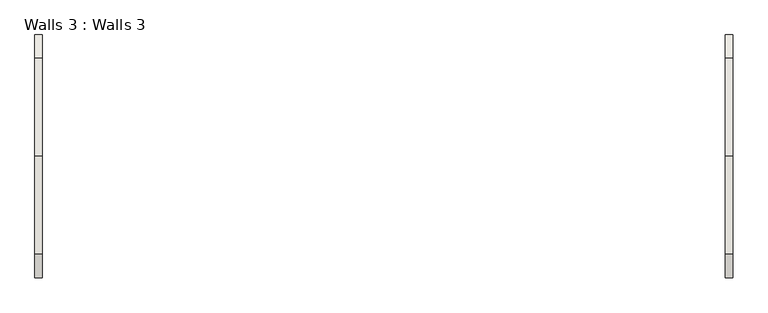
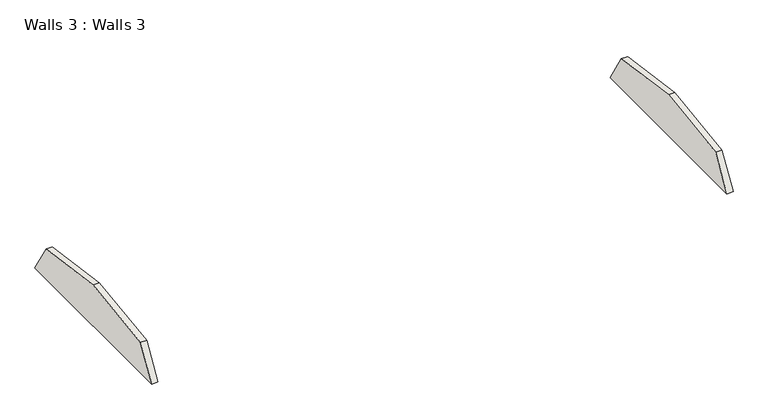
"""IFC4 building model written with IfcOpenShell, lengths in millimetres: wall geometry, Walls 3 : Walls 3."""

from ifc_helpers import new_model, si_unit, frame, origin, place, context, project, spatial, polyline, outline, extrude, source, transform, mapped, element, save


def walls_3_walls_3_da5502db(model_context):
    return source(origin(), model_context, "Body", "SweptSolid", [
        extrude(outline(polyline([(7113.2615366, 4718.0467955), (10133.2027784, 4305.4367595), (10859.8068451, 3111.5), (3366.7162281, 3111.5), (4093.3202949, 4305.4367595), (7113.2615366, 4718.0467955)])), frame((28804.3870052, 0.0, 0.0), z_axis=(1.0, 0.0, 0.0), x_axis=(0.0, 1.0, 0.0)), (0.0, 0.0, 1.0), 228.6),
        extrude(outline(polyline([(7113.2615366, 4718.0467955), (10133.2027784, 4305.4367595), (10859.8068451, 3111.5), (3366.7162281, 3111.5), (4093.3202949, 4305.4367595), (7113.2615366, 4718.0467955)])), frame((7500.1370052, 0.0, 0.0), z_axis=(1.0, 0.0, 0.0), x_axis=(0.0, 1.0, 0.0)), (0.0, 0.0, 1.0), 228.6),
    ])


if __name__ == "__main__":
    model = new_model("IFC4")
    model_context = context("Model", 3, world=origin())
    ifc_project = project(units=[si_unit("LENGTHUNIT", "METRE", prefix="MILLI")], contexts=[model_context])
    site = spatial("IfcSite", under=ifc_project)
    building = spatial("IfcBuilding", under=site)
    placement = place(None, origin())
    walls_3_walls_3_shape = walls_3_walls_3_da5502db(model_context)
    element("IfcWall", 1, ObjectType="Walls 3 : Walls 3", at=placement, inside=building, context=model_context, shape_type="MappedRepresentation", body=[
        mapped(walls_3_walls_3_shape, transform((0.0, 0.0, 0.0), x_axis=(1.0, 0.0, 0.0), y_axis=(0.0, 1.0, 0.0), z_axis=(0.0, 0.0, 1.0))),
    ])
    save(model, "model.ifc")

# Revit data of these elements
# Element 1 (IfcWall, "Walls 3 : Walls 3")
#   Materials on its faces: "Default Wall"
# Materials
#   "Default Wall": class "Miscellaneous", colour RGB 80 80 80, transparency 0
